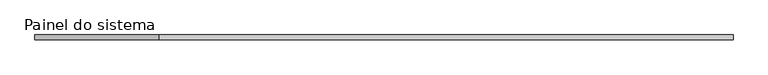
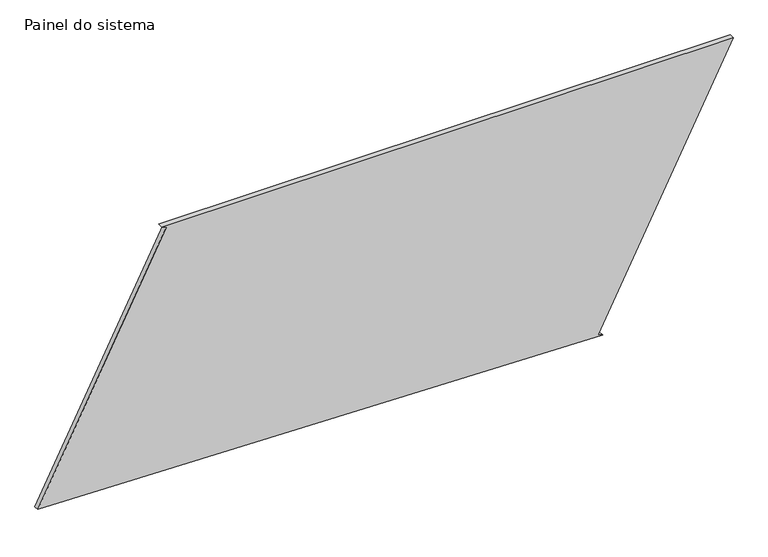
"""IFC4 building model written with IfcOpenShell, lengths in millimetres: plate geometry, Painel do sistema : Envidraçado."""

from ifc_helpers import new_model, si_unit, frame, origin, place, context, project, spatial, polyline, outline, extrude, source, transform, mapped, element, save


def painel_do_sistema_52fbb16d(model_context):
    return source(origin(), model_context, "Body", "SweptSolid", [
        extrude(outline(polyline([(0.0, 1084.9586338), (11.291819, 1062.6540418), (1343.8925663, 1737.2902952), (1343.8925663, -1118.2079553), (1332.6007473, -1095.9033633), (65.6769784, -1737.2902952), (0.0, 1084.9586338)])), frame((0.0, 24.5, 0.0), z_axis=(0.0, 1.0, 0.0), x_axis=(0.0, 0.0, 1.0)), (0.0, 0.0, 1.0), 25.0),
    ])


if __name__ == "__main__":
    model = new_model("IFC4")
    model_context = context("Model", 3, world=origin())
    ifc_project = project(units=[si_unit("LENGTHUNIT", "METRE", prefix="MILLI")], contexts=[model_context])
    site = spatial("IfcSite", under=ifc_project)
    building = spatial("IfcBuilding", under=site)
    placement = place(None, origin())
    painel_do_sistema_shape = painel_do_sistema_52fbb16d(model_context)
    element("IfcPlate", 1, ObjectType="Painel do sistema : Envidraçado", at=placement, inside=building, context=model_context, shape_type="MappedRepresentation", body=[
        mapped(painel_do_sistema_shape, transform((0.0, 0.0, 0.0), x_axis=(1.0, 0.0, 0.0), y_axis=(0.0, 1.0, 0.0), z_axis=(0.0, 0.0, 1.0))),
    ])
    save(model, "model.ifc")

# Revit data of these elements
# Type "Painel do sistema : Envidraçado"
#   Construction Type Id = "GSP4R"
#   Analytic Construction = "Vidraça única Pilkington 1/8 pol"
#   Visual Light Transmittance = 0.9
#   Solar Heat Gain Coefficient = 0.86
#   Heat Transfer Coefficient (U) = 6.7069 W/(m²·K)
# Element 1 (IfcPlate, "Painel do sistema : Envidraçado")
#   Materials on its faces: "Vidro"
# Materials
#   "Vidro": class "Vidro", colour RGB 0 128 192, transparency 0.9, Description = "Vidro de sílica", Cost = 0
